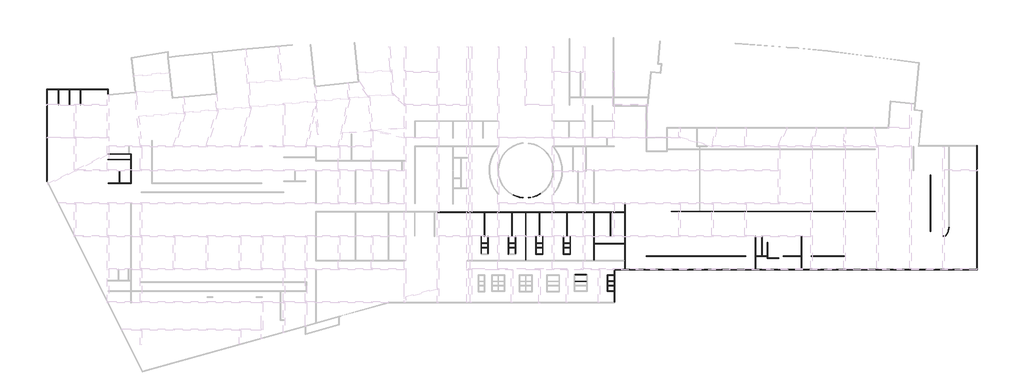
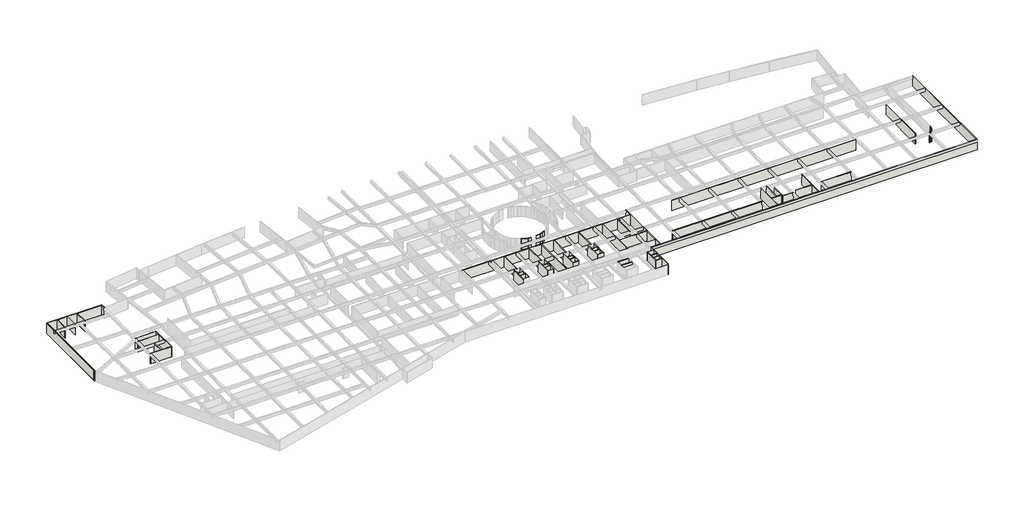
# One storey, part 2 of 8: 71 walls.
"""IFC4 building model written with IfcOpenShell, lengths in millimetres."""

from ifc_helpers import new_model, si_unit, origin, origin_with_axes, place, context, project, spatial, polyline, outline, extrude, faceted_brep, element, save

model = new_model("IFC4")

# Units and contexts
model_context = context("Model", 3, world=origin())
ifc_project = project(units=[si_unit("LENGTHUNIT", "METRE", prefix="MILLI")], contexts=[model_context])

# Site, building, storey
site = spatial("IfcSite", under=ifc_project)
building = spatial("IfcBuilding", under=site)
storey = spatial("IfcBuildingStorey", under=building, Name="户型图", Elevation=0.0)

# Walls
placement = place(None, origin())
element("IfcWall", 1, ObjectType="所有墙体", at=placement, inside=storey, context=model_context, shape_type="Brep", body=[
    faceted_brep([(299643.8653576, 28778.6264659, 0.0), (299643.8653576, 3574.4623872, 0.0), (299643.8653576, 3574.4623872, 3300.0), (299643.8653576, 28778.6264659, 3300.0), (299763.8653576, 28778.6264659, 0.0), (299763.8653576, 28778.6264659, 3300.0), (299763.8653576, 28658.6264659, 3300.0), (299763.8653576, 3602.7905445, 3300.0), (299763.8653576, 3334.4623872, 3300.0), (299763.8653576, 3334.4623872, 0.0), (299763.8653576, 3602.7905445, 0.0), (299763.8653576, 28658.6264659, 0.0)], [[[0, 1, 2, 3]], [[4, 5, 6, 7, 8, 9, 10, 11]], [[1, 0, 4, 11, 10, 9]], [[3, 2, 8, 7, 6, 5]], [[2, 1, 9, 8]], [[0, 3, 5, 4]]]),
])
element("IfcWall", 2, ObjectType="所有墙体", at=placement, inside=storey, context=model_context, shape_type="Brep", body=[
    faceted_brep([(454678.7450641, -29507.78226, 0.0), (454678.7450641, -20627.78226, 0.0), (454678.7450641, -20507.78226, 0.0), (454678.7450641, -20507.78226, 3300.0), (454678.7450641, -20627.78226, 3300.0), (454678.7450641, -29507.78226, 3300.0), (454558.7450641, -29507.78226, 0.0), (454558.7450641, -29507.78226, 3300.0), (454558.7450641, -26471.3735096, 3300.0), (454558.7450641, -26351.3735096, 3300.0), (454558.7450641, -25021.6891861, 3300.0), (454558.7450641, -24901.6891861, 3300.0), (454558.7450641, -23771.6182304, 3300.0), (454558.7450641, -23651.6182304, 3300.0), (454558.7450641, -22071.3735096, 3300.0), (454558.7450641, -21951.3735096, 3300.0), (454558.7450641, -20507.78226, 3300.0), (454558.7450641, -20507.78226, 0.0), (454558.7450641, -21951.3735096, 0.0), (454558.7450641, -22071.3735096, 0.0), (454558.7450641, -23651.6182304, 0.0), (454558.7450641, -23771.6182304, 0.0), (454558.7450641, -24901.6891861, 0.0), (454558.7450641, -25021.6891861, 0.0), (454558.7450641, -26351.3735096, 0.0), (454558.7450641, -26471.3735096, 0.0)], [[[0, 1, 2, 3, 4, 5]], [[6, 7, 8, 9, 10, 11, 12, 13, 14, 15, 16, 17, 18, 19, 20, 21, 22, 23, 24, 25]], [[2, 1, 0, 6, 25, 24, 23, 22, 21, 20, 19, 18, 17]], [[5, 4, 3, 16, 15, 14, 13, 12, 11, 10, 9, 8, 7]], [[0, 5, 7, 6]], [[3, 2, 17, 16]]]),
])
element("IfcWall", 3, ObjectType="所有墙体", at=placement, inside=storey, context=model_context, shape_type="Brep", body=[
    faceted_brep([(454678.7450641, -20627.78226, 0.0), (553578.7450641, -20627.78226, 0.0), (553578.7450641, -20627.78226, 3300.0), (454678.7450641, -20627.78226, 3300.0), (454678.7450641, -20507.78226, 0.0), (454678.7450641, -20507.78226, 3300.0), (457393.8653576, -20507.78226, 3300.0), (457513.8653576, -20507.78226, 3300.0), (505543.8653576, -20507.78226, 3300.0), (505663.8653576, -20507.78226, 3300.0), (553458.7450641, -20507.78226, 3300.0), (553578.7450641, -20507.78226, 3300.0), (553578.7450641, -20507.78226, 0.0), (553458.7450641, -20507.78226, 0.0), (505663.8653576, -20507.78226, 0.0), (505543.8653576, -20507.78226, 0.0), (457513.8653576, -20507.78226, 0.0), (457393.8653576, -20507.78226, 0.0)], [[[0, 1, 2, 3]], [[4, 5, 6, 7, 8, 9, 10, 11, 12, 13, 14, 15, 16, 17]], [[1, 0, 4, 17, 16, 15, 14, 13, 12]], [[3, 2, 11, 10, 9, 8, 7, 6, 5]], [[0, 3, 5, 4]], [[2, 1, 12, 11]]]),
])
element("IfcWall", 4, ObjectType="所有墙体", at=placement, inside=storey, context=model_context, shape_type="Brep", body=[
    faceted_brep([(553578.7450641, -20507.78226, 0.0), (553578.7450641, 13292.21774, 0.0), (553578.7450641, 13292.21774, 3300.0), (553578.7450641, -20507.78226, 3300.0), (553458.7450641, -20507.78226, 0.0), (553458.7450641, -20507.78226, 3300.0), (553458.7450641, 13172.21774, 3300.0), (553458.7450641, 13292.21774, 3300.0), (553458.7450641, 13292.21774, 0.0), (553458.7450641, 13172.21774, 0.0)], [[[0, 1, 2, 3]], [[4, 5, 6, 7, 8, 9]], [[1, 0, 4, 9, 8]], [[3, 2, 7, 6, 5]], [[0, 3, 5, 4]], [[2, 1, 8, 7]]]),
])
element("IfcWall", 5, ObjectType="所有墙体", at=placement, inside=storey, context=model_context, shape_type="Brep", body=[
    faceted_brep([(316365.2591436, 27278.6306619, 0.0), (316365.2591436, 28778.6264659, 0.0), (316365.2591436, 28778.6264659, 3300.0), (316365.2591436, 27278.6306619, 3300.0), (316245.2591436, 27267.272828, 0.0), (316245.2591436, 27267.272828, 3300.0), (316245.2591436, 28658.6264659, 3300.0), (316245.2591436, 28778.6264659, 3300.0), (316245.2591436, 28778.6264659, 0.0), (316245.2591436, 28658.6264659, 0.0)], [[[0, 1, 2, 3]], [[4, 5, 6, 7, 8, 9]], [[1, 0, 4, 9, 8]], [[3, 2, 7, 6, 5]], [[0, 3, 5, 4]], [[2, 1, 8, 7]]]),
])
element("IfcWall", 6, ObjectType="所有墙体", at=placement, inside=storey, context=model_context, shape_type="Brep", body=[
    faceted_brep([(316245.2591436, 28778.6264659, 0.0), (299763.8653576, 28778.6264659, 0.0), (299763.8653576, 28778.6264659, 3300.0), (316245.2591436, 28778.6264659, 3300.0), (316245.2591436, 28658.6264659, 0.0), (316245.2591436, 28658.6264659, 3300.0), (308913.8653576, 28658.6264659, 3300.0), (308793.8653576, 28658.6264659, 3300.0), (305913.8653576, 28658.6264659, 3300.0), (305793.8653576, 28658.6264659, 3300.0), (302913.8653576, 28658.6264659, 3300.0), (302793.8653576, 28658.6264659, 3300.0), (299763.8653576, 28658.6264659, 3300.0), (299763.8653576, 28658.6264659, 0.0), (302793.8653576, 28658.6264659, 0.0), (302913.8653576, 28658.6264659, 0.0), (305793.8653576, 28658.6264659, 0.0), (305913.8653576, 28658.6264659, 0.0), (308793.8653576, 28658.6264659, 0.0), (308913.8653576, 28658.6264659, 0.0)], [[[0, 1, 2, 3]], [[4, 5, 6, 7, 8, 9, 10, 11, 12, 13, 14, 15, 16, 17, 18, 19]], [[1, 0, 4, 19, 18, 17, 16, 15, 14, 13]], [[3, 2, 12, 11, 10, 9, 8, 7, 6, 5]], [[0, 3, 5, 4]], [[2, 1, 13, 12]]]),
])
element("IfcWall", 7, ObjectType="所有墙体", at=placement, inside=storey, context=model_context, shape_type="SweptSolid", body=[
    extrude(outline(polyline([(299643.8653576, 3842.7905446), (299643.8653576, 28658.6264659), (299763.8653576, 28658.6264659), (299763.8653576, 3602.7905445), (299643.8653576, 3842.7905446)])), origin_with_axes(), (0.0, 0.0, 1.0), 3300.0),
])
element("IfcWall", 8, ObjectType="所有墙体", at=placement, inside=storey, context=model_context, shape_type="Brep", body=[
    faceted_brep([(406353.8653576, -4921.3735096, 0.0), (419043.8653576, -4921.3735096, 0.0), (419163.8653576, -4921.3735096, 0.0), (426543.8653576, -4921.3735096, 0.0), (426663.8653576, -4921.3735096, 0.0), (430293.8653576, -4921.3735096, 0.0), (430413.8653576, -4921.3735096, 0.0), (434043.8653576, -4921.3735096, 0.0), (434163.8653576, -4921.3735096, 0.0), (441543.8653576, -4921.3735096, 0.0), (441663.8653576, -4921.3735096, 0.0), (448893.8653567, -4921.3735096, 0.0), (449013.8653567, -4921.3735096, 0.0), (453393.8653577, -4921.3735096, 0.0), (453513.8653577, -4921.3735096, 0.0), (457393.8653576, -4921.3735096, 0.0), (457393.8653576, -4921.3735096, 3300.0), (453513.8653577, -4921.3735096, 3300.0), (453393.8653577, -4921.3735096, 3300.0), (449013.8653567, -4921.3735096, 3300.0), (448893.8653567, -4921.3735096, 3300.0), (441663.8653576, -4921.3735096, 3300.0), (441543.8653576, -4921.3735096, 3300.0), (434163.8653576, -4921.3735096, 3300.0), (434043.8653576, -4921.3735096, 3300.0), (430413.8653576, -4921.3735096, 3300.0), (430293.8653576, -4921.3735096, 3300.0), (426663.8653576, -4921.3735096, 3300.0), (426543.8653576, -4921.3735096, 3300.0), (419163.8653576, -4921.3735096, 3300.0), (419043.8653576, -4921.3735096, 3300.0), (406353.8653576, -4921.3735096, 3300.0), (406353.8653576, -4801.3735096, 0.0), (406353.8653576, -4801.3735096, 3300.0), (457393.8653576, -4801.3735096, 3300.0), (457393.8653576, -4801.3735096, 0.0)], [[[0, 1, 2, 3, 4, 5, 6, 7, 8, 9, 10, 11, 12, 13, 14, 15, 16, 17, 18, 19, 20, 21, 22, 23, 24, 25, 26, 27, 28, 29, 30, 31]], [[32, 33, 34, 35]], [[15, 14, 13, 12, 11, 10, 9, 8, 7, 6, 5, 4, 3, 2, 1, 0, 32, 35]], [[31, 30, 29, 28, 27, 26, 25, 24, 23, 22, 21, 20, 19, 18, 17, 16, 34, 33]], [[0, 31, 33, 32]], [[16, 15, 35, 34]]]),
])
element("IfcWall", 9, ObjectType="所有墙体", at=placement, inside=storey, context=model_context, shape_type="Brep", body=[
    faceted_brep([(457513.8653576, -20507.78226, 0.0), (457513.8653576, -2461.3735096, 0.0), (457513.8653576, -2461.3735096, 3300.0), (457513.8653576, -20507.78226, 3300.0), (457393.8653576, -20507.78226, 0.0), (457393.8653576, -20507.78226, 3300.0), (457393.8653576, -18121.3735105, 3300.0), (457393.8653576, -18001.3735105, 3300.0), (457393.8653576, -13521.3735106, 3300.0), (457393.8653576, -13401.3735106, 3300.0), (457393.8653576, -4921.3735096, 3300.0), (457393.8653576, -4801.3735096, 3300.0), (457393.8653576, -2461.3735096, 3300.0), (457393.8653576, -2461.3735096, 0.0), (457393.8653576, -4801.3735096, 0.0), (457393.8653576, -4921.3735096, 0.0), (457393.8653576, -13401.3735106, 0.0), (457393.8653576, -13521.3735106, 0.0), (457393.8653576, -18001.3735105, 0.0), (457393.8653576, -18121.3735105, 0.0)], [[[0, 1, 2, 3]], [[4, 5, 6, 7, 8, 9, 10, 11, 12, 13, 14, 15, 16, 17, 18, 19]], [[1, 0, 4, 19, 18, 17, 16, 15, 14, 13]], [[2, 1, 13, 12]], [[3, 2, 12, 11, 10, 9, 8, 7, 6, 5]], [[0, 3, 5, 4]]]),
])
element("IfcWall", 10, ObjectType="所有墙体", at=placement, inside=storey, context=model_context, shape_type="SweptSolid", body=[
    extrude(outline(polyline([(430413.8653576, -4921.3735096), (430413.8653576, -18001.3735105), (430293.8653576, -18001.3735105), (430293.8653576, -4921.3735096), (430413.8653576, -4921.3735096)])), origin_with_axes(), (0.0, 0.0, 1.0), 3300.0),
])
element("IfcWall", 11, ObjectType="所有墙体", at=placement, inside=storey, context=model_context, shape_type="SweptSolid", body=[
    extrude(outline(polyline([(426543.8653576, -11461.3735096), (426543.8653576, -4921.3735096), (426663.8653576, -4921.3735096), (426663.8653576, -11461.3735096), (426543.8653576, -11461.3735096)])), origin_with_axes(), (0.0, 0.0, 1.0), 3300.0),
])
element("IfcWall", 12, ObjectType="所有墙体", at=placement, inside=storey, context=model_context, shape_type="SweptSolid", body=[
    extrude(outline(polyline([(434043.8653576, -11361.3735096), (434043.8653576, -4921.3735096), (434163.8653576, -4921.3735096), (434163.8653576, -11361.3735096), (434043.8653576, -11361.3735096)])), origin_with_axes(), (0.0, 0.0, 1.0), 3300.0),
])
element("IfcWall", 13, ObjectType="所有墙体", at=placement, inside=storey, context=model_context, shape_type="SweptSolid", body=[
    extrude(outline(polyline([(441543.8653576, -11461.3735096), (441543.8653576, -4921.3735096), (441663.8653576, -4921.3735096), (441663.8653576, -11461.3735096), (441543.8653576, -11461.3735096)])), origin_with_axes(), (0.0, 0.0, 1.0), 3300.0),
])
element("IfcWall", 14, ObjectType="所有墙体", at=placement, inside=storey, context=model_context, shape_type="Brep", body=[
    faceted_brep([(448893.8653567, -4921.3735096, 0.0), (448893.8653567, -18001.3735105, 0.0), (448893.8653567, -18001.3735105, 3300.0), (448893.8653567, -4921.3735096, 3300.0), (449013.8653567, -4921.3735096, 0.0), (449013.8653567, -4921.3735096, 3300.0), (449013.8653567, -13401.3735106, 3300.0), (449013.8653567, -13521.3735106, 3300.0), (449013.8653567, -18001.3735105, 3300.0), (449013.8653567, -18001.3735105, 0.0), (449013.8653567, -13521.3735106, 0.0), (449013.8653567, -13401.3735106, 0.0)], [[[0, 1, 2, 3]], [[4, 5, 6, 7, 8, 9, 10, 11]], [[1, 0, 4, 11, 10, 9]], [[3, 2, 8, 7, 6, 5]], [[0, 3, 5, 4]], [[2, 1, 9, 8]]]),
])
element("IfcWall", 15, ObjectType="所有墙体", at=placement, inside=storey, context=model_context, shape_type="SweptSolid", body=[
    extrude(outline(polyline([(453393.8653577, -11461.3735096), (453393.8653577, -4921.3735096), (453513.8653577, -4921.3735096), (453513.8653577, -11461.3735096), (453393.8653577, -11461.3735096)])), origin_with_axes(), (0.0, 0.0, 1.0), 3300.0),
])
element("IfcWall", 16, ObjectType="所有墙体", at=placement, inside=storey, context=model_context, shape_type="SweptSolid", body=[
    extrude(outline(polyline([(457393.8653576, -13521.3735106), (449013.8653567, -13521.3735106), (449013.8653567, -13401.3735106), (457393.8653576, -13401.3735106), (457393.8653576, -13521.3735106)])), origin_with_axes(), (0.0, 0.0, 1.0), 3300.0),
])
element("IfcWall", 17, ObjectType="所有墙体", at=placement, inside=storey, context=model_context, shape_type="Brep", body=[
    faceted_brep([(440643.8653631, -11461.3735096, 0.0), (440643.8653631, -16421.3261103, 0.0), (440643.8653631, -16421.3261103, 3300.0), (440643.8653631, -11461.3735096, 3300.0), (440763.8653631, -11461.3735096, 0.0), (440763.8653631, -11461.3735096, 3300.0), (440763.8653631, -13301.0813645, 3300.0), (440763.8653631, -13421.0813645, 3300.0), (440763.8653631, -14501.0813645, 3300.0), (440763.8653631, -14621.0813645, 3300.0), (440763.8653631, -16301.3261103, 3300.0), (440763.8653631, -16421.3261103, 3300.0), (440763.8653631, -16421.3261103, 0.0), (440763.8653631, -16301.3261103, 0.0), (440763.8653631, -14621.0813645, 0.0), (440763.8653631, -14501.0813645, 0.0), (440763.8653631, -13421.0813645, 0.0), (440763.8653631, -13301.0813645, 0.0)], [[[0, 1, 2, 3]], [[4, 5, 6, 7, 8, 9, 10, 11, 12, 13, 14, 15, 16, 17]], [[1, 0, 4, 17, 16, 15, 14, 13, 12]], [[3, 2, 11, 10, 9, 8, 7, 6, 5]], [[0, 3, 5, 4]], [[2, 1, 12, 11]]]),
])
element("IfcWall", 18, ObjectType="所有墙体", at=placement, inside=storey, context=model_context, shape_type="Brep", body=[
    faceted_brep([(440763.8653631, -16421.3261103, 0.0), (442563.8653631, -16421.3261103, 0.0), (442563.8653631, -16421.3261103, 3300.0), (440763.8653631, -16421.3261103, 3300.0), (440763.8653631, -16301.3261103, 0.0), (440763.8653631, -16301.3261103, 3300.0), (442443.8653631, -16301.3261103, 3300.0), (442563.8653631, -16301.3261103, 3300.0), (442563.8653631, -16301.3261103, 0.0), (442443.8653631, -16301.3261103, 0.0)], [[[0, 1, 2, 3]], [[4, 5, 6, 7, 8, 9]], [[1, 0, 4, 9, 8]], [[3, 2, 7, 6, 5]], [[0, 3, 5, 4]], [[2, 1, 8, 7]]]),
])
element("IfcWall", 19, ObjectType="所有墙体", at=placement, inside=storey, context=model_context, shape_type="Brep", body=[
    faceted_brep([(442563.8653631, -16301.3261103, 0.0), (442563.8653631, -11461.3735096, 0.0), (442563.8653631, -11461.3735096, 3300.0), (442563.8653631, -16301.3261103, 3300.0), (442443.8653631, -16301.3261103, 0.0), (442443.8653631, -16301.3261103, 3300.0), (442443.8653631, -14621.0813645, 3300.0), (442443.8653631, -14501.0813645, 3300.0), (442443.8653631, -13421.0813645, 3300.0), (442443.8653631, -13301.0813645, 3300.0), (442443.8653631, -11461.3735096, 3300.0), (442443.8653631, -11461.3735096, 0.0), (442443.8653631, -13301.0813645, 0.0), (442443.8653631, -13421.0813645, 0.0), (442443.8653631, -14501.0813645, 0.0), (442443.8653631, -14621.0813645, 0.0)], [[[0, 1, 2, 3]], [[4, 5, 6, 7, 8, 9, 10, 11, 12, 13, 14, 15]], [[1, 0, 4, 15, 14, 13, 12, 11]], [[2, 1, 11, 10]], [[3, 2, 10, 9, 8, 7, 6, 5]], [[0, 3, 5, 4]]]),
])
element("IfcWall", 20, ObjectType="所有墙体", at=placement, inside=storey, context=model_context, shape_type="SweptSolid", body=[
    extrude(outline(polyline([(442443.8653631, -13421.0813645), (440763.8653631, -13421.0813645), (440763.8653631, -13301.0813645), (442443.8653631, -13301.0813645), (442443.8653631, -13421.0813645)])), origin_with_axes(), (0.0, 0.0, 1.0), 3300.0),
])
element("IfcWall", 21, ObjectType="所有墙体", at=placement, inside=storey, context=model_context, shape_type="SweptSolid", body=[
    extrude(outline(polyline([(440763.8653631, -14501.0813645), (442443.8653631, -14501.0813645), (442443.8653631, -14621.0813645), (440763.8653631, -14621.0813645), (440763.8653631, -14501.0813645)])), origin_with_axes(), (0.0, 0.0, 1.0), 3300.0),
])
element("IfcWall", 22, ObjectType="所有墙体", at=placement, inside=storey, context=model_context, shape_type="Brep", body=[
    faceted_brep([(433143.8653576, -11461.3735096, 0.0), (433143.8653576, -16421.3261103, 0.0), (433143.8653576, -16421.3261103, 3300.0), (433143.8653576, -11461.3735096, 3300.0), (433263.8653576, -11461.3735096, 0.0), (433263.8653576, -11461.3735096, 3300.0), (433263.8653576, -13301.0813645, 3300.0), (433263.8653576, -13421.0813645, 3300.0), (433263.8653576, -14501.0813645, 3300.0), (433263.8653576, -14621.0813645, 3300.0), (433263.8653576, -16301.3261103, 3300.0), (433263.8653576, -16421.3261103, 3300.0), (433263.8653576, -16421.3261103, 0.0), (433263.8653576, -16301.3261103, 0.0), (433263.8653576, -14621.0813645, 0.0), (433263.8653576, -14501.0813645, 0.0), (433263.8653576, -13421.0813645, 0.0), (433263.8653576, -13301.0813645, 0.0)], [[[0, 1, 2, 3]], [[4, 5, 6, 7, 8, 9, 10, 11, 12, 13, 14, 15, 16, 17]], [[1, 0, 4, 17, 16, 15, 14, 13, 12]], [[3, 2, 11, 10, 9, 8, 7, 6, 5]], [[0, 3, 5, 4]], [[2, 1, 12, 11]]]),
])
element("IfcWall", 23, ObjectType="所有墙体", at=placement, inside=storey, context=model_context, shape_type="Brep", body=[
    faceted_brep([(433263.8653576, -16421.3261103, 0.0), (435063.8653576, -16421.3261103, 0.0), (435063.8653576, -16421.3261103, 3300.0), (433263.8653576, -16421.3261103, 3300.0), (433263.8653576, -16301.3261103, 0.0), (433263.8653576, -16301.3261103, 3300.0), (434943.8653576, -16301.3261103, 3300.0), (435063.8653576, -16301.3261103, 3300.0), (435063.8653576, -16301.3261103, 0.0), (434943.8653576, -16301.3261103, 0.0)], [[[0, 1, 2, 3]], [[4, 5, 6, 7, 8, 9]], [[1, 0, 4, 9, 8]], [[3, 2, 7, 6, 5]], [[0, 3, 5, 4]], [[2, 1, 8, 7]]]),
])
element("IfcWall", 24, ObjectType="所有墙体", at=placement, inside=storey, context=model_context, shape_type="Brep", body=[
    faceted_brep([(434943.8653576, -11461.3735096, 0.0), (434943.8653576, -13301.0813645, 0.0), (434943.8653576, -13421.0813645, 0.0), (434943.8653576, -14501.0813645, 0.0), (434943.8653576, -14621.0813645, 0.0), (434943.8653576, -16301.3261103, 0.0), (434943.8653576, -16301.3261103, 3300.0), (434943.8653576, -14621.0813645, 3300.0), (434943.8653576, -14501.0813645, 3300.0), (434943.8653576, -13421.0813645, 3300.0), (434943.8653576, -13301.0813645, 3300.0), (434943.8653576, -11461.3735096, 3300.0), (435063.8653576, -11461.3735096, 0.0), (435063.8653576, -11461.3735096, 3300.0), (435063.8653576, -16301.3261103, 3300.0), (435063.8653576, -16301.3261103, 0.0)], [[[0, 1, 2, 3, 4, 5, 6, 7, 8, 9, 10, 11]], [[12, 13, 14, 15]], [[5, 4, 3, 2, 1, 0, 12, 15]], [[11, 10, 9, 8, 7, 6, 14, 13]], [[0, 11, 13, 12]], [[6, 5, 15, 14]]]),
])
element("IfcWall", 25, ObjectType="所有墙体", at=placement, inside=storey, context=model_context, shape_type="SweptSolid", body=[
    extrude(outline(polyline([(434943.8653576, -14621.0813645), (433263.8653576, -14621.0813645), (433263.8653576, -14501.0813645), (434943.8653576, -14501.0813645), (434943.8653576, -14621.0813645)])), origin_with_axes(), (0.0, 0.0, 1.0), 3300.0),
])
element("IfcWall", 26, ObjectType="所有墙体", at=placement, inside=storey, context=model_context, shape_type="SweptSolid", body=[
    extrude(outline(polyline([(433263.8653576, -13301.0813645), (434943.8653576, -13301.0813645), (434943.8653576, -13421.0813645), (433263.8653576, -13421.0813645), (433263.8653576, -13301.0813645)])), origin_with_axes(), (0.0, 0.0, 1.0), 3300.0),
])
element("IfcWall", 27, ObjectType="所有墙体", at=placement, inside=storey, context=model_context, shape_type="Brep", body=[
    faceted_brep([(425643.8653576, -11461.3735096, 0.0), (425643.8653576, -16421.3735096, 0.0), (425643.8653576, -16421.3735096, 3300.0), (425643.8653576, -11461.3735096, 3300.0), (425763.8653576, -11461.3735096, 0.0), (425763.8653576, -11461.3735096, 3300.0), (425763.8653576, -13301.0813645, 3300.0), (425763.8653576, -13421.0813645, 3300.0), (425763.8653576, -14501.0813645, 3300.0), (425763.8653576, -14621.0813645, 3300.0), (425763.8653576, -16301.3735096, 3300.0), (425763.8653576, -16421.3735096, 3300.0), (425763.8653576, -16421.3735096, 0.0), (425763.8653576, -16301.3735096, 0.0), (425763.8653576, -14621.0813645, 0.0), (425763.8653576, -14501.0813645, 0.0), (425763.8653576, -13421.0813645, 0.0), (425763.8653576, -13301.0813645, 0.0)], [[[0, 1, 2, 3]], [[4, 5, 6, 7, 8, 9, 10, 11, 12, 13, 14, 15, 16, 17]], [[1, 0, 4, 17, 16, 15, 14, 13, 12]], [[3, 2, 11, 10, 9, 8, 7, 6, 5]], [[0, 3, 5, 4]], [[2, 1, 12, 11]]]),
])
element("IfcWall", 28, ObjectType="所有墙体", at=placement, inside=storey, context=model_context, shape_type="Brep", body=[
    faceted_brep([(427563.8653576, -16301.3735096, 0.0), (427563.8653576, -11461.3735096, 0.0), (427563.8653576, -11461.3735096, 3300.0), (427563.8653576, -16301.3735096, 3300.0), (427443.8653576, -16301.3735096, 0.0), (427443.8653576, -16301.3735096, 3300.0), (427443.8653576, -13421.0813645, 3300.0), (427443.8653576, -13301.0813645, 3300.0), (427443.8653576, -11461.3735096, 3300.0), (427443.8653576, -11461.3735096, 0.0), (427443.8653576, -13301.0813645, 0.0), (427443.8653576, -13421.0813645, 0.0)], [[[0, 1, 2, 3]], [[4, 5, 6, 7, 8, 9, 10, 11]], [[1, 0, 4, 11, 10, 9]], [[2, 1, 9, 8]], [[3, 2, 8, 7, 6, 5]], [[0, 3, 5, 4]]]),
])
element("IfcWall", 29, ObjectType="所有墙体", at=placement, inside=storey, context=model_context, shape_type="SweptSolid", body=[
    extrude(outline(polyline([(427443.8653576, -13421.0813645), (425763.8653576, -13421.0813645), (425763.8653576, -13301.0813645), (427443.8653576, -13301.0813645), (427443.8653576, -13421.0813645)])), origin_with_axes(), (0.0, 0.0, 1.0), 3300.0),
])
element("IfcWall", 30, ObjectType="所有墙体", at=placement, inside=storey, context=model_context, shape_type="Brep", body=[
    faceted_brep([(427443.8653576, -13421.0813645, 0.0), (427443.8653576, -14501.0813645, 0.0), (427443.8653576, -14621.0813645, 0.0), (427443.8653576, -14621.0813645, 3300.0), (427443.8653576, -14501.0813645, 3300.0), (427443.8653576, -13421.0813645, 3300.0), (427563.8653576, -13421.0813645, 0.0), (427563.8653576, -13421.0813645, 3300.0), (427563.8653576, -14621.0813645, 3300.0), (427563.8653576, -14621.0813645, 0.0)], [[[0, 1, 2, 3, 4, 5]], [[6, 7, 8, 9]], [[2, 1, 0, 6, 9]], [[5, 4, 3, 8, 7]], [[0, 5, 7, 6]], [[3, 2, 9, 8]]]),
])
element("IfcWall", 31, ObjectType="所有墙体", at=placement, inside=storey, context=model_context, shape_type="SweptSolid", body=[
    extrude(outline(polyline([(427443.8653576, -14621.0813645), (425763.8653576, -14621.0813645), (425763.8653576, -14501.0813645), (427443.8653576, -14501.0813645), (427443.8653576, -14621.0813645)])), origin_with_axes(), (0.0, 0.0, 1.0), 3300.0),
])
element("IfcWall", 32, ObjectType="所有墙体", at=placement, inside=storey, context=model_context, shape_type="Brep", body=[
    faceted_brep([(418143.8653576, -11461.3735096, 0.0), (418143.8653576, -16421.3261103, 0.0), (418143.8653576, -16421.3261103, 3300.0), (418143.8653576, -11461.3735096, 3300.0), (418263.8653576, -11461.3735096, 0.0), (418263.8653576, -11461.3735096, 3300.0), (418263.8653576, -13301.0813645, 3300.0), (418263.8653576, -13421.0813645, 3300.0), (418263.8653576, -14501.0813645, 3300.0), (418263.8653576, -14621.0813645, 3300.0), (418263.8653576, -16301.3261103, 3300.0), (418263.8653576, -16421.3261103, 3300.0), (418263.8653576, -16421.3261103, 0.0), (418263.8653576, -16301.3261103, 0.0), (418263.8653576, -14621.0813645, 0.0), (418263.8653576, -14501.0813645, 0.0), (418263.8653576, -13421.0813645, 0.0), (418263.8653576, -13301.0813645, 0.0)], [[[0, 1, 2, 3]], [[4, 5, 6, 7, 8, 9, 10, 11, 12, 13, 14, 15, 16, 17]], [[1, 0, 4, 17, 16, 15, 14, 13, 12]], [[3, 2, 11, 10, 9, 8, 7, 6, 5]], [[0, 3, 5, 4]], [[2, 1, 12, 11]]]),
])
element("IfcWall", 33, ObjectType="所有墙体", at=placement, inside=storey, context=model_context, shape_type="Brep", body=[
    faceted_brep([(420063.8653576, -16301.3261103, 0.0), (420063.8653576, -11461.3735096, 0.0), (420063.8653576, -11461.3735096, 3300.0), (420063.8653576, -16301.3261103, 3300.0), (419943.8653576, -16301.3261103, 0.0), (419943.8653576, -16301.3261103, 3300.0), (419943.8653576, -14621.0813645, 3300.0), (419943.8653576, -14501.0813645, 3300.0), (419943.8653576, -13421.0813645, 3300.0), (419943.8653576, -13301.0813645, 3300.0), (419943.8653576, -11461.3735096, 3300.0), (419943.8653576, -11461.3735096, 0.0), (419943.8653576, -13301.0813645, 0.0), (419943.8653576, -13421.0813645, 0.0), (419943.8653576, -14501.0813645, 0.0), (419943.8653576, -14621.0813645, 0.0)], [[[0, 1, 2, 3]], [[4, 5, 6, 7, 8, 9, 10, 11, 12, 13, 14, 15]], [[1, 0, 4, 15, 14, 13, 12, 11]], [[2, 1, 11, 10]], [[3, 2, 10, 9, 8, 7, 6, 5]], [[0, 3, 5, 4]]]),
])
element("IfcWall", 34, ObjectType="所有墙体", at=placement, inside=storey, context=model_context, shape_type="SweptSolid", body=[
    extrude(outline(polyline([(419943.8653576, -13421.0813645), (418263.8653576, -13421.0813645), (418263.8653576, -13301.0813645), (419943.8653576, -13301.0813645), (419943.8653576, -13421.0813645)])), origin_with_axes(), (0.0, 0.0, 1.0), 3300.0),
])
element("IfcWall", 35, ObjectType="所有墙体", at=placement, inside=storey, context=model_context, shape_type="SweptSolid", body=[
    extrude(outline(polyline([(418263.8653576, -14501.0813645), (419943.8653576, -14501.0813645), (419943.8653576, -14621.0813645), (418263.8653576, -14621.0813645), (418263.8653576, -14501.0813645)])), origin_with_axes(), (0.0, 0.0, 1.0), 3300.0),
])
element("IfcWall", 36, ObjectType="所有墙体", at=placement, inside=storey, context=model_context, shape_type="SweptSolid", body=[
    extrude(outline(polyline([(443713.8653655, -21921.3735096), (446993.8653655, -21921.3735096), (446993.8653655, -22041.3735096), (443713.8653655, -22041.3735096), (443713.8653655, -21921.3735096)])), origin_with_axes(), (0.0, 0.0, 1.0), 3300.0),
])
element("IfcWall", 37, ObjectType="所有墙体", at=placement, inside=storey, context=model_context, shape_type="SweptSolid", body=[
    extrude(outline(polyline([(446993.8653655, -23821.6182553), (443713.8653655, -23821.6182553), (443713.8653655, -23701.6182553), (446993.8653655, -23701.6182553), (446993.8653655, -23821.6182553)])), origin_with_axes(), (0.0, 0.0, 1.0), 3300.0),
])
element("IfcWall", 38, ObjectType="所有墙体", at=placement, inside=storey, context=model_context, shape_type="Brep", body=[
    faceted_brep([(454558.7450641, -21951.3735096, 0.0), (452658.7450641, -21951.3735096, 0.0), (452658.7450641, -21951.3735096, 3300.0), (454558.7450641, -21951.3735096, 3300.0), (454558.7450641, -22071.3735096, 0.0), (454558.7450641, -22071.3735096, 3300.0), (452778.7450641, -22071.3735096, 3300.0), (452658.7450641, -22071.3735096, 3300.0), (452658.7450641, -22071.3735096, 0.0), (452778.7450641, -22071.3735096, 0.0)], [[[0, 1, 2, 3]], [[4, 5, 6, 7, 8, 9]], [[1, 0, 4, 9, 8]], [[3, 2, 7, 6, 5]], [[0, 3, 5, 4]], [[2, 1, 8, 7]]]),
])
element("IfcWall", 39, ObjectType="所有墙体", at=placement, inside=storey, context=model_context, shape_type="Brep", body=[
    faceted_brep([(452658.7450641, -22071.3735096, 0.0), (452658.7450641, -26471.3735096, 0.0), (452658.7450641, -26471.3735096, 3300.0), (452658.7450641, -22071.3735096, 3300.0), (452778.7450641, -22071.3735096, 0.0), (452778.7450641, -22071.3735096, 3300.0), (452778.7450641, -23651.6182304, 3300.0), (452778.7450641, -23771.6182304, 3300.0), (452778.7450641, -24901.6891861, 3300.0), (452778.7450641, -25021.6891861, 3300.0), (452778.7450641, -26351.3735096, 3300.0), (452778.7450641, -26471.3735096, 3300.0), (452778.7450641, -26471.3735096, 0.0), (452778.7450641, -26351.3735096, 0.0), (452778.7450641, -25021.6891861, 0.0), (452778.7450641, -24901.6891861, 0.0), (452778.7450641, -23771.6182304, 0.0), (452778.7450641, -23651.6182304, 0.0)], [[[0, 1, 2, 3]], [[4, 5, 6, 7, 8, 9, 10, 11, 12, 13, 14, 15, 16, 17]], [[1, 0, 4, 17, 16, 15, 14, 13, 12]], [[3, 2, 11, 10, 9, 8, 7, 6, 5]], [[0, 3, 5, 4]], [[2, 1, 12, 11]]]),
])
element("IfcWall", 40, ObjectType="所有墙体", at=placement, inside=storey, context=model_context, shape_type="SweptSolid", body=[
    extrude(outline(polyline([(454558.7450641, -26471.3735096), (452778.7450641, -26471.3735096), (452778.7450641, -26351.3735096), (454558.7450641, -26351.3735096), (454558.7450641, -26471.3735096)])), origin_with_axes(), (0.0, 0.0, 1.0), 3300.0),
])
element("IfcWall", 41, ObjectType="所有墙体", at=placement, inside=storey, context=model_context, shape_type="SweptSolid", body=[
    extrude(outline(polyline([(454558.7450641, -23771.6182304), (452778.7450641, -23771.6182304), (452778.7450641, -23651.6182304), (454558.7450641, -23651.6182304), (454558.7450641, -23771.6182304)])), origin_with_axes(), (0.0, 0.0, 1.0), 3300.0),
])
element("IfcWall", 42, ObjectType="所有墙体", at=placement, inside=storey, context=model_context, shape_type="SweptSolid", body=[
    extrude(outline(polyline([(452778.7450641, -24901.6891861), (454558.7450641, -24901.6891861), (454558.7450641, -25021.6891861), (452778.7450641, -25021.6891861), (452778.7450641, -24901.6891861)])), origin_with_axes(), (0.0, 0.0, 1.0), 3300.0),
])
element("IfcWall", 43, ObjectType="所有墙体", at=placement, inside=storey, context=model_context, shape_type="Brep", body=[
    faceted_brep([(470077.8817886, -4720.6191139, 0.0), (525777.8817886, -4720.6191139, 0.0), (525777.8817886, -4720.6191139, 3300.0), (470077.8817886, -4720.6191139, 3300.0), (470077.8817886, -4600.6191139, 0.0), (470077.8817886, -4600.6191139, 3300.0), (477798.5776142, -4600.6191139, 3300.0), (477918.5776142, -4600.6191139, 3300.0), (525777.8817886, -4600.6191139, 3300.0), (525777.8817886, -4600.6191139, 0.0), (477918.5776142, -4600.6191139, 0.0), (477798.5776142, -4600.6191139, 0.0)], [[[0, 1, 2, 3]], [[4, 5, 6, 7, 8, 9, 10, 11]], [[1, 0, 4, 11, 10, 9]], [[2, 1, 9, 8]], [[3, 2, 8, 7, 6, 5]], [[0, 3, 5, 4]]]),
])
element("IfcWall", 44, ObjectType="所有墙体", at=placement, inside=storey, context=model_context, shape_type="SweptSolid", body=[
    extrude(outline(polyline([(540793.8653576, -10161.3735096), (540793.8653576, 5238.6264883), (540913.8653576, 5238.6264883), (540913.8653576, -10161.3735096), (540793.8653576, -10161.3735096)])), origin_with_axes(), (0.0, 0.0, 1.0), 3300.0),
])
element("IfcWall", 45, ObjectType="所有墙体", at=placement, inside=storey, context=model_context, shape_type="SweptSolid", body=[
    extrude(outline(polyline([(545622.62401, -10027.282131), (545793.8653576, -9056.1241898), (545913.8653576, -9066.6228294), (545737.8103499, -10065.0803941), (545622.62401, -10027.282131)])), origin_with_axes(), (0.0, 0.0, 1.0), 3300.0),
])
element("IfcWall", 46, ObjectType="所有墙体", at=placement, inside=storey, context=model_context, shape_type="SweptSolid", body=[
    extrude(outline(polyline([(545273.5733736, -10732.4668565), (545622.62401, -10027.282131), (545737.8103499, -10065.0803941), (545377.0865502, -10793.8483352), (545273.5733736, -10732.4668565)])), origin_with_axes(), (0.0, 0.0, 1.0), 3300.0),
])
element("IfcWall", 47, ObjectType="所有墙体", at=placement, inside=storey, context=model_context, shape_type="Brep", body=[
    faceted_brep([(545273.5733736, -10732.4668565, 0.0), (544938.9052501, -11210.4224701, 0.0), (544825.0403579, -11373.0383888, 0.0), (544825.0403579, -11373.0383888, 3300.0), (544938.9052501, -11210.4224701, 3300.0), (545273.5733736, -10732.4668565, 3300.0), (545377.0865502, -10793.8483352, 0.0), (545377.0865502, -10793.8483352, 3300.0), (545014.0455969, -11312.3245491, 3300.0), (545014.0455969, -11312.3245491, 0.0)], [[[0, 1, 2, 3, 4, 5]], [[6, 7, 8, 9]], [[2, 1, 0, 6, 9]], [[5, 4, 3, 8, 7]], [[0, 5, 7, 6]], [[3, 2, 9, 8]]]),
])
element("IfcWall", 48, ObjectType="所有墙体", at=placement, inside=storey, context=model_context, shape_type="SweptSolid", body=[
    extrude(outline(polyline([(544335.5151741, -11404.2484646), (544938.9052501, -11210.4224701), (544825.0403579, -11373.0383888), (544372.2155412, -11518.4985546), (544335.5151741, -11404.2484646)])), origin_with_axes(), (0.0, 0.0, 1.0), 3300.0),
])
element("IfcWall", 49, ObjectType="所有墙体", at=placement, inside=storey, context=model_context, shape_type="Brep", body=[
    faceted_brep([(499453.8653576, -17401.3735096, 0.0), (496413.8653576, -17401.3735096, 0.0), (496293.8653576, -17401.3735096, 0.0), (496293.8653576, -17401.3735096, 3300.0), (496413.8653576, -17401.3735096, 3300.0), (499453.8653576, -17401.3735096, 3300.0), (499453.8653576, -17521.3735096, 0.0), (499453.8653576, -17521.3735096, 3300.0), (496293.8653576, -17521.3735096, 3300.0), (496293.8653576, -17521.3735096, 0.0)], [[[0, 1, 2, 3, 4, 5]], [[6, 7, 8, 9]], [[2, 1, 0, 6, 9]], [[5, 4, 3, 8, 7]], [[0, 5, 7, 6]], [[3, 2, 9, 8]]]),
])
element("IfcWall", 50, ObjectType="所有墙体", at=placement, inside=storey, context=model_context, shape_type="Brep", body=[
    faceted_brep([(496413.8653576, -17401.3735096, 0.0), (496413.8653576, -13161.3735096, 0.0), (496413.8653576, -13161.3735096, 3300.0), (496413.8653576, -17401.3735096, 3300.0), (496293.8653576, -17401.3735096, 0.0), (496293.8653576, -17401.3735096, 3300.0), (496293.8653576, -16921.3735096, 3300.0), (496293.8653576, -16801.3735096, 3300.0), (496293.8653576, -13161.3735096, 3300.0), (496293.8653576, -13161.3735096, 0.0), (496293.8653576, -16801.3735096, 0.0), (496293.8653576, -16921.3735096, 0.0)], [[[0, 1, 2, 3]], [[4, 5, 6, 7, 8, 9, 10, 11]], [[1, 0, 4, 11, 10, 9]], [[2, 1, 9, 8]], [[3, 2, 8, 7, 6, 5]], [[0, 3, 5, 4]]]),
])
element("IfcWall", 51, ObjectType="所有墙体", at=placement, inside=storey, context=model_context, shape_type="Brep", body=[
    faceted_brep([(496293.8653576, -16801.3735096, 0.0), (494913.8653447, -16801.3735096, 0.0), (494793.8653447, -16801.3735096, 0.0), (493163.8653576, -16801.3735096, 0.0), (493163.8653576, -16801.3735096, 3300.0), (494793.8653447, -16801.3735096, 3300.0), (494913.8653447, -16801.3735096, 3300.0), (496293.8653576, -16801.3735096, 3300.0), (496293.8653576, -16921.3735096, 0.0), (496293.8653576, -16921.3735096, 3300.0), (493163.8653576, -16921.3735096, 3300.0), (493163.8653576, -16921.3735096, 0.0)], [[[0, 1, 2, 3, 4, 5, 6, 7]], [[8, 9, 10, 11]], [[3, 2, 1, 0, 8, 11]], [[7, 6, 5, 4, 10, 9]], [[0, 7, 9, 8]], [[4, 3, 11, 10]]]),
])
element("IfcWall", 52, ObjectType="所有墙体", at=placement, inside=storey, context=model_context, shape_type="Brep", body=[
    faceted_brep([(493163.8653576, -20461.3735096, 0.0), (493163.8653576, -16921.3735096, 0.0), (493163.8653576, -16801.3735096, 0.0), (493163.8653576, -11461.3735096, 0.0), (493163.8653576, -11461.3735096, 3300.0), (493163.8653576, -16801.3735096, 3300.0), (493163.8653576, -16921.3735096, 3300.0), (493163.8653576, -20461.3735096, 3300.0), (493043.8653576, -20461.3735096, 0.0), (493043.8653576, -20461.3735096, 3300.0), (493043.8653576, -11461.3735096, 3300.0), (493043.8653576, -11461.3735096, 0.0)], [[[0, 1, 2, 3, 4, 5, 6, 7]], [[8, 9, 10, 11]], [[3, 2, 1, 0, 8, 11]], [[4, 3, 11, 10]], [[7, 6, 5, 4, 10, 9]], [[0, 7, 9, 8]]]),
])
element("IfcWall", 53, ObjectType="所有墙体", at=placement, inside=storey, context=model_context, shape_type="SweptSolid", body=[
    extrude(outline(polyline([(494793.8653447, -16801.3735096), (494793.8653447, -11461.3735096), (494913.8653447, -11461.3735096), (494913.8653447, -16801.3735096), (494793.8653447, -16801.3735096)])), origin_with_axes(), (0.0, 0.0, 1.0), 3300.0),
])
element("IfcWall", 54, ObjectType="所有墙体", at=placement, inside=storey, context=model_context, shape_type="SweptSolid", body=[
    extrude(outline(polyline([(463253.8653576, -16801.3735096), (490353.8653576, -16801.3735096), (490353.8653576, -16921.3735096), (463253.8653576, -16921.3735096), (463253.8653576, -16801.3735096)])), origin_with_axes(), (0.0, 0.0, 1.0), 3300.0),
])
element("IfcWall", 55, ObjectType="所有墙体", at=placement, inside=storey, context=model_context, shape_type="SweptSolid", body=[
    extrude(outline(polyline([(419043.8653576, -11461.3735096), (419043.8653576, -4921.3735096), (419163.8653576, -4921.3735096), (419163.8653576, -11461.3735096), (419043.8653576, -11461.3735096)])), origin_with_axes(), (0.0, 0.0, 1.0), 3300.0),
])
element("IfcWall", 56, ObjectType="所有墙体", at=placement, inside=storey, context=model_context, shape_type="SweptSolid", body=[
    extrude(outline(polyline([(428646.1033058, -826.2003992), (426928.370024, -200.9966142), (426979.2779354, -91.8242459), (428676.6752117, -709.6263303), (428646.1033058, -826.2003992)])), origin_with_axes(), (0.0, 0.0, 1.0), 3300.0),
])
element("IfcWall", 57, ObjectType="所有墙体", at=placement, inside=storey, context=model_context, shape_type="SweptSolid", body=[
    extrude(outline(polyline([(429594.0759942, -982.9685352), (428646.1033058, -826.2003992), (428676.6752117, -709.6263303), (429613.654721, -864.5765023), (429594.0759942, -982.9685352)])), origin_with_axes(), (0.0, 0.0, 1.0), 3300.0),
])
element("IfcWall", 58, ObjectType="所有墙体", at=placement, inside=storey, context=model_context, shape_type="SweptSolid", body=[
    extrude(outline(polyline([(432353.0023323, -752.4483166), (431114.8378153, -982.760697), (431092.8929, -864.7843405), (432321.8852813, -636.1780794), (432353.0023323, -752.4483166)])), origin_with_axes(), (0.0, 0.0, 1.0), 3300.0),
])
element("IfcWall", 59, ObjectType="所有墙体", at=placement, inside=storey, context=model_context, shape_type="SweptSolid", body=[
    extrude(outline(polyline([(433370.9449586, -393.4084462), (432353.0023323, -752.4483166), (432321.8852813, -636.1780794), (433323.0051881, -283.0717723), (433370.9449586, -393.4084462)])), origin_with_axes(), (0.0, 0.0, 1.0), 3300.0),
])
element("IfcWall", 60, ObjectType="所有墙体", at=placement, inside=storey, context=model_context, shape_type="SweptSolid", body=[
    extrude(outline(polyline([(434310.2990917, 96.4273342), (433370.9449586, -393.4084462), (433323.0051881, -283.0717723), (434248.2402677, 199.4014838), (434310.2990917, 96.4273342)])), origin_with_axes(), (0.0, 0.0, 1.0), 3300.0),
])
element("IfcWall", 61, ObjectType="所有墙体", at=placement, inside=storey, context=model_context, shape_type="Brep", body=[
    faceted_brep([(316353.7983208, 10978.5928116, 0.0), (322593.8653576, 10978.6261687, 0.0), (322713.8653576, 10978.6268101, 0.0), (322713.8653576, 10978.6268101, 3300.0), (322593.8653576, 10978.6261687, 3300.0), (316353.7983208, 10978.5928116, 3300.0), (316353.7976793, 11098.5928116, 0.0), (316353.7976793, 11098.5928116, 3300.0), (321993.8653557, 11098.6229613, 3300.0), (322113.8653557, 11098.6236028, 3300.0), (322713.8653576, 11098.6268101, 3300.0), (322713.8653576, 11098.6268101, 0.0), (322113.8653557, 11098.6236028, 0.0), (321993.8653557, 11098.6229613, 0.0)], [[[0, 1, 2, 3, 4, 5]], [[6, 7, 8, 9, 10, 11, 12, 13]], [[2, 1, 0, 6, 13, 12, 11]], [[5, 4, 3, 10, 9, 8, 7]], [[0, 5, 7, 6]], [[3, 2, 11, 10]]]),
])
element("IfcWall", 62, ObjectType="所有墙体", at=placement, inside=storey, context=model_context, shape_type="Brep", body=[
    faceted_brep([(322593.8653576, 10978.6261687, 0.0), (322593.8653576, 9598.6264904, 0.0), (322593.8653576, 9478.6264904, 0.0), (322593.8653576, 3098.6264904, 0.0), (322593.8653576, 2978.6264904, 0.0), (322593.8653576, 2978.6264904, 3300.0), (322593.8653576, 3098.6264904, 3300.0), (322593.8653576, 9478.6264904, 3300.0), (322593.8653576, 9598.6264904, 3300.0), (322593.8653576, 10978.6261687, 3300.0), (322713.8653576, 10978.6268101, 0.0), (322713.8653576, 10978.6268101, 3300.0), (322713.8653576, 2978.6264904, 3300.0), (322713.8653576, 2978.6264904, 0.0)], [[[0, 1, 2, 3, 4, 5, 6, 7, 8, 9]], [[10, 11, 12, 13]], [[4, 3, 2, 1, 0, 10, 13]], [[9, 8, 7, 6, 5, 12, 11]], [[0, 9, 11, 10]], [[5, 4, 13, 12]]]),
])
element("IfcWall", 63, ObjectType="所有墙体", at=placement, inside=storey, context=model_context, shape_type="SweptSolid", body=[
    extrude(outline(polyline([(316253.8653576, 9598.6264904), (322593.8653576, 9598.6264904), (322593.8653576, 9478.6264904), (316253.8653576, 9478.6264904), (316253.8653576, 9598.6264904)])), origin_with_axes(), (0.0, 0.0, 1.0), 3300.0),
])
element("IfcWall", 64, ObjectType="所有墙体", at=placement, inside=storey, context=model_context, shape_type="SweptSolid", body=[
    extrude(outline(polyline([(302913.8653576, 28658.6264659), (302913.8653576, 24538.6264904), (302793.8653576, 24538.6264904), (302793.8653576, 28658.6264659), (302913.8653576, 28658.6264659)])), origin_with_axes(), (0.0, 0.0, 1.0), 3300.0),
])
element("IfcWall", 65, ObjectType="所有墙体", at=placement, inside=storey, context=model_context, shape_type="SweptSolid", body=[
    extrude(outline(polyline([(305793.8653576, 24438.6264659), (305793.8653576, 28658.6264659), (305913.8653576, 28658.6264659), (305913.8653576, 24438.6264659), (305793.8653576, 24438.6264659)])), origin_with_axes(), (0.0, 0.0, 1.0), 3300.0),
])
element("IfcWall", 66, ObjectType="所有墙体", at=placement, inside=storey, context=model_context, shape_type="SweptSolid", body=[
    extrude(outline(polyline([(308913.8653576, 28658.6264659), (308913.8653576, 24538.6264904), (308793.8653576, 24538.6264904), (308793.8653576, 28658.6264659), (308913.8653576, 28658.6264659)])), origin_with_axes(), (0.0, 0.0, 1.0), 3300.0),
])
element("IfcWall", 67, ObjectType="所有墙体", at=placement, inside=storey, context=model_context, shape_type="Brep", body=[
    faceted_brep([(322593.8653576, 3098.6264904, 0.0), (319563.8653576, 3098.6264904, 0.0), (319443.8653576, 3098.6264904, 0.0), (316353.8653576, 3098.6264904, 0.0), (316353.8653576, 3098.6264904, 3300.0), (319443.8653576, 3098.6264904, 3300.0), (319563.8653576, 3098.6264904, 3300.0), (322593.8653576, 3098.6264904, 3300.0), (322593.8653576, 2978.6264904, 0.0), (322593.8653576, 2978.6264904, 3300.0), (316353.8653576, 2978.6264904, 3300.0), (316353.8653576, 2978.6264904, 0.0)], [[[0, 1, 2, 3, 4, 5, 6, 7]], [[8, 9, 10, 11]], [[3, 2, 1, 0, 8, 11]], [[4, 3, 11, 10]], [[7, 6, 5, 4, 10, 9]], [[0, 7, 9, 8]]]),
])
element("IfcWall", 68, ObjectType="所有墙体", at=placement, inside=storey, context=model_context, shape_type="SweptSolid", body=[
    extrude(outline(polyline([(319443.8653576, 3098.6264904), (319443.8653576, 6438.6264883), (319563.8653576, 6438.6264883), (319563.8653576, 3098.6264904), (319443.8653576, 3098.6264904)])), origin_with_axes(), (0.0, 0.0, 1.0), 3300.0),
])
element("IfcWall", 69, ObjectType="所有墙体", at=placement, inside=storey, context=model_context, shape_type="Brep", body=[
    faceted_brep([(505543.8653576, -11361.373495, 0.0), (505543.8653576, -16801.3735096, 0.0), (505543.8653576, -16921.3735096, 0.0), (505543.8653576, -20507.78226, 0.0), (505543.8653576, -20507.78226, 3300.0), (505543.8653576, -16921.3735096, 3300.0), (505543.8653576, -16801.3735096, 3300.0), (505543.8653576, -11361.373495, 3300.0), (505663.8653576, -11361.373495, 0.0), (505663.8653576, -11361.373495, 3300.0), (505663.8653576, -20507.78226, 3300.0), (505663.8653576, -20507.78226, 0.0)], [[[0, 1, 2, 3, 4, 5, 6, 7]], [[8, 9, 10, 11]], [[3, 2, 1, 0, 8, 11]], [[7, 6, 5, 4, 10, 9]], [[0, 7, 9, 8]], [[4, 3, 11, 10]]]),
])
element("IfcWall", 70, ObjectType="所有墙体", at=placement, inside=storey, context=model_context, shape_type="SweptSolid", body=[
    extrude(outline(polyline([(500653.8653576, -16801.3735096), (505543.8653576, -16801.3735096), (505543.8653576, -16921.3735096), (500653.8653576, -16921.3735096), (500653.8653576, -16801.3735096)])), origin_with_axes(), (0.0, 0.0, 1.0), 3300.0),
])
element("IfcWall", 71, ObjectType="所有墙体", at=placement, inside=storey, context=model_context, shape_type="SweptSolid", body=[
    extrude(outline(polyline([(517353.8653576, -16921.3735096), (508353.8653576, -16921.3735096), (508353.8653576, -16801.3735096), (517353.8653576, -16801.3735096), (517353.8653576, -16921.3735096)])), origin_with_axes(), (0.0, 0.0, 1.0), 3300.0),
])

save(model, "model.ifc")

# Revit data of these elements
# Type "所有墙体"
#   Layers, outside or top first: 120 mm "默认" (function 1)
# Elements 1, 2, 3, 4, 5, 6, 7, 8, 9, 10, 11, 12, 13, 14, 15, 16, 17, 18, 19, 20, 21, 22, 23, 24, 25, 26, 27, 28, 29, 30, 31, 32, 33, 34, 35, 36, 37, 38, 39, 40, 41, 42, 43, 44, 45, 46, 47, 48, 49, 50, 51, 52, 53, 54, 55, 56, 57, 58, 59, 60, 61, 62, 63, 64, 65, 66, 67, 68, 69, 70, 71 (IfcWall, "所有墙体")
#   Top Offset = 0 mm
#   Base Offset = 0 mm
#   wall height = 3300 mm
#   Phase Created = 新构造
#   Base Constraint = 户型图
#   Top Constraint = 层高
#   Materials on its faces: "默认"
# Materials
#   "默认": class "其他", colour RGB 192 192 192, transparency 0, Cost = 0
